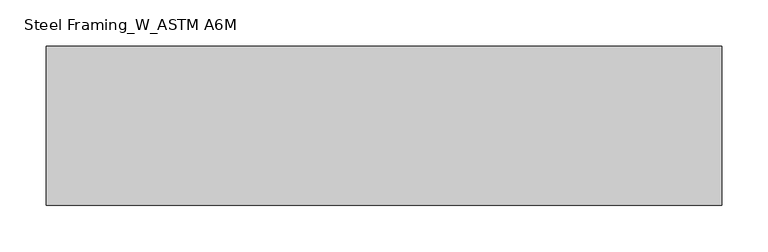
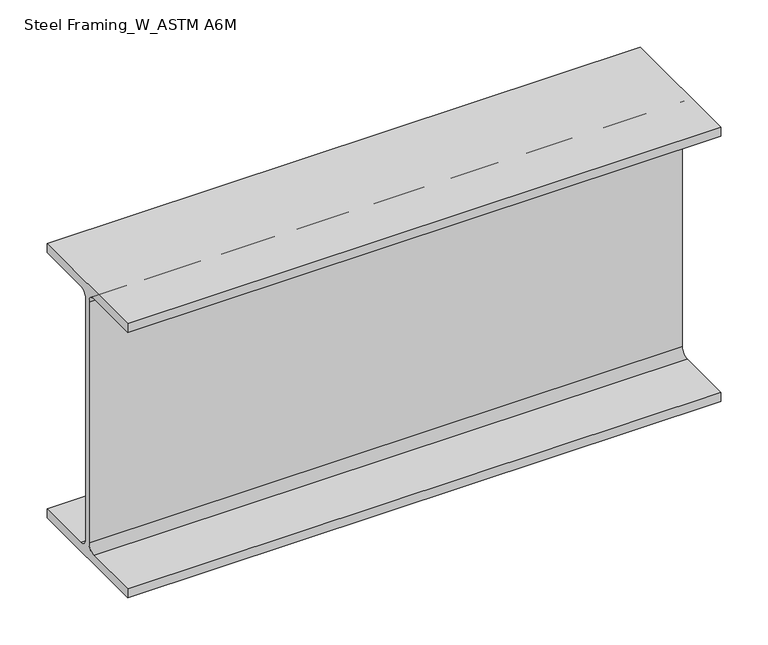
"""IFC4 building model written with IfcOpenShell, lengths in millimetres: beam geometry, Steel Framing_W_ASTM A6M : H_SB_AR_S02_W360x51_RG1."""

import ifcopenshell
import ifcopenshell.guid

model = None  # the IFC model being written
_history = None  # IfcOwnerHistory: only IFC2X3 demands one
_inside = {}  # id of a spatial element -> (the spatial element, [elements in it])
_under = {}  # id of a project, library or spatial element -> (it, [spatial elements below it])
_declared = {}  # id of a project -> (the project, [libraries it declares])
_typed = {}  # id of a type object -> (the type object, [elements of that type])
_made_of = {}  # id of a material, layer set ... -> (it, [elements and type objects made of it])


def new_model(schema):
    """Start an empty IFC model of exactly this schema.

    Asked for "IFC4X3", IfcOpenShell would pick the latest addendum, in which some entities
    have other attributes; the version numbers below select the first issue.
    IFC2X3 requires an IfcOwnerHistory on every rooted entity: one is made here for all.
    """
    global model, _history
    if schema == "IFC4X3":
        model = ifcopenshell.file(schema_version=(4, 3, 0, 0))
    else:
        model = ifcopenshell.file(schema=schema)
    _inside.clear()
    _under.clear()
    _declared.clear()
    _typed.clear()
    _made_of.clear()
    _history = None
    if model.schema == "IFC2X3":
        org = make("IfcOrganization", Name="unknown")
        user = make(
            "IfcPersonAndOrganization",
            ThePerson=make("IfcPerson", FamilyName="unknown"),
            TheOrganization=org,
        )
        app = make(
            "IfcApplication",
            ApplicationDeveloper=org,
            Version="unknown",
            ApplicationFullName="unknown",
            ApplicationIdentifier="unknown",
        )
        _history = make(
            "IfcOwnerHistory",
            OwningUser=user,
            OwningApplication=app,
            ChangeAction="ADDED",
            CreationDate=0,
        )
    return model


def make(cls, **values):
    """One entity of the class cls with the attributes given. An attribute that is None is left unset."""
    return model.create_entity(
        cls, **{name: value for name, value in values.items() if value is not None}
    )


def rooted(cls, **values):
    """An entity with a GlobalId (a new one), such as an element, a storey or a relation."""
    return make(cls, GlobalId=ifcopenshell.guid.new(), OwnerHistory=_history, **values)


def si_unit(unit_type, name, prefix=None):
    """IfcSIUnit, for example si_unit("LENGTHUNIT", "METRE", prefix="MILLI")."""
    return make("IfcSIUnit", UnitType=unit_type, Prefix=prefix, Name=name)


def assignment(units):
    """IfcUnitAssignment: the units of a project."""
    return None if units is None else make("IfcUnitAssignment", Units=units)


def point(xyz):
    """IfcCartesianPoint."""
    return None if xyz is None else make("IfcCartesianPoint", Coordinates=xyz)


def direction(xyz):
    """IfcDirection."""
    return None if xyz is None else make("IfcDirection", DirectionRatios=xyz)


def frame(location, z_axis=None, x_axis=None):
    """IfcAxis2Placement3D, a coordinate frame: its origin and axes. An axis left out is left unset."""
    return make(
        "IfcAxis2Placement3D",
        Location=point(location),
        Axis=direction(z_axis),
        RefDirection=direction(x_axis),
    )


def frame_2d(location, x_axis=None):
    """IfcAxis2Placement2D, a coordinate frame in the plane: its origin and x axis."""
    return make(
        "IfcAxis2Placement2D", Location=point(location), RefDirection=direction(x_axis)
    )


def origin():
    """The frame at (0, 0, 0) with its axes left unset."""
    return frame((0.0, 0.0, 0.0))


def place(relative_to, where):
    """IfcLocalPlacement: puts the frame where relative to a parent placement (None: the world)."""
    return make(
        "IfcLocalPlacement", PlacementRelTo=relative_to, RelativePlacement=where
    )


def context(
    kind, dimensions, precision=None, world=None, true_north=None, identifier=None
):
    """IfcGeometricRepresentationContext, for example the 3D "Model" context."""
    return make(
        "IfcGeometricRepresentationContext",
        ContextIdentifier=identifier,
        ContextType=kind,
        CoordinateSpaceDimension=dimensions,
        Precision=precision,
        WorldCoordinateSystem=world,
        TrueNorth=true_north,
    )


def project(units=None, contexts=None):
    """IfcProject with its units and contexts."""
    return rooted(
        "IfcProject",
        Name="project",
        RepresentationContexts=contexts,
        UnitsInContext=assignment(units),
    )


def spatial(cls, under=None, at=None, **own):
    """A site, building, storey or space (cls), placed at a placement, below another one or the project."""
    s = rooted(cls, ObjectPlacement=at, **own)
    if under is not None:
        _under.setdefault(under.id(), (under, []))[1].append(s)
    return s


def polyline(points):
    """IfcPolyline through the points."""
    return make("IfcPolyline", Points=[point(p) for p in points])


def circle_curve(where, radius):
    """IfcCircle in the frame where."""
    return make("IfcCircle", Position=where, Radius=radius)


def trimmed(basis, trim1, trim2, sense, master):
    """IfcTrimmedCurve: the piece of a basis curve between two trims."""
    return make(
        "IfcTrimmedCurve",
        BasisCurve=basis,
        Trim1=trim1,
        Trim2=trim2,
        SenseAgreement=sense,
        MasterRepresentation=master,
    )


def segment(curve, same_sense, transition):
    """IfcCompositeCurveSegment."""
    return make(
        "IfcCompositeCurveSegment",
        Transition=transition,
        SameSense=same_sense,
        ParentCurve=curve,
    )


def composite_curve(segments, self_intersect=None):
    """IfcCompositeCurve: segments joined end to end."""
    return make("IfcCompositeCurve", Segments=segments, SelfIntersect=self_intersect)


def outline(outer, holes=None, kind="AREA"):
    """IfcArbitraryClosedProfileDef: a profile drawn as a closed curve; with holes, ...WithVoids."""
    if holes is None:
        return make("IfcArbitraryClosedProfileDef", ProfileType=kind, OuterCurve=outer)
    return make(
        "IfcArbitraryProfileDefWithVoids",
        ProfileType=kind,
        OuterCurve=outer,
        InnerCurves=holes,
    )


def extrude(swept, where, along, depth):
    """IfcExtrudedAreaSolid: the profile swept, set in the frame where, extruded along a direction by depth."""
    return make(
        "IfcExtrudedAreaSolid",
        SweptArea=swept,
        Position=where,
        ExtrudedDirection=direction(along),
        Depth=depth,
    )


def shape(context_of_items, identifier, shape_type, items):
    """IfcShapeRepresentation: the items that make up one representation, for example the "Body"."""
    return make(
        "IfcShapeRepresentation",
        ContextOfItems=context_of_items,
        RepresentationIdentifier=identifier,
        RepresentationType=shape_type,
        Items=items,
    )


def source(mapping_origin, context_of_items, identifier, shape_type, items):
    """IfcRepresentationMap: a shape defined once, which mapped items show again and again."""
    return make(
        "IfcRepresentationMap",
        MappingOrigin=mapping_origin,
        MappedRepresentation=shape(context_of_items, identifier, shape_type, items),
    )


def transform(
    local_origin,
    x_axis=None,
    y_axis=None,
    z_axis=None,
    scale=None,
    scale2=None,
    scale3=None,
    uniform=True,
):
    """IfcCartesianTransformationOperator3D, or its non-uniform kind. x_axis, y_axis, z_axis: its Axis1, 2, 3."""
    if uniform:
        return make(
            "IfcCartesianTransformationOperator3D",
            Axis1=direction(x_axis),
            Axis2=direction(y_axis),
            LocalOrigin=point(local_origin),
            Scale=scale,
            Axis3=direction(z_axis),
        )
    return make(
        "IfcCartesianTransformationOperator3DnonUniform",
        Axis1=direction(x_axis),
        Axis2=direction(y_axis),
        LocalOrigin=point(local_origin),
        Scale=scale,
        Axis3=direction(z_axis),
        Scale2=scale2,
        Scale3=scale3,
    )


def mapped(mapping_source, mapping_target):
    """IfcMappedItem: shows the shape of a source again, moved by a transform."""
    return make(
        "IfcMappedItem", MappingSource=mapping_source, MappingTarget=mapping_target
    )


def made_of(thing, what):
    """Note that an element or type object is made of a material, layer set ...; save() writes the relation."""
    if what is not None:
        _made_of.setdefault(what.id(), (what, []))[1].append(thing)
    return thing


def element(
    cls,
    number,
    at=None,
    inside=None,
    cuts=None,
    type_object=None,
    material=None,
    context=None,
    identifier="Body",
    shape_type=None,
    held_by="IfcProductDefinitionShape",
    body=None,
    shapes=None,
    **own,
):
    """One element of the class cls, such as IfcWall. Its Tag is "e" and its number.

    at: its placement. inside: the storey or other place that contains it. cuts: it is an
    opening in that element (IfcRelVoidsElement). A single representation is given by context,
    identifier, shape_type and body (its items); several are given by shapes. held_by: the class
    of the entity that holds the representations. save() writes the other relations.
    """
    e = rooted(cls, Tag="e%d" % number, ObjectPlacement=at, **own)
    if body is not None:
        shapes = [shape(context, identifier, shape_type, body)]
    if shapes is not None:
        e.Representation = make(held_by, Representations=shapes)
    if inside is not None:
        _inside.setdefault(inside.id(), (inside, []))[1].append(e)
    if cuts is not None:
        rooted(
            "IfcRelVoidsElement", RelatingBuildingElement=cuts, RelatedOpeningElement=e
        )
    if type_object is not None:
        _typed.setdefault(type_object.id(), (type_object, []))[1].append(e)
    return made_of(e, material)


def aggregate(whole, parts):
    """IfcRelAggregates: a whole, such as a stair, and the parts it consists of."""
    return rooted("IfcRelAggregates", RelatingObject=whole, RelatedObjects=parts)


def save(model, path):
    """Write the relations noted so far, then the file.

    IfcRelAggregates (storeys below a building ...), IfcRelContainedInSpatialStructure (elements
    in a storey), IfcRelDefinesByType, IfcRelAssociatesMaterial and IfcRelDeclares: one each for
    every whole, place, type object, material and project.
    """
    for whole, parts in _under.values():
        aggregate(whole, parts)
    for where, things in _inside.values():
        rooted(
            "IfcRelContainedInSpatialStructure",
            RelatedElements=things,
            RelatingStructure=where,
        )
    for kind, things in _typed.values():
        rooted("IfcRelDefinesByType", RelatedObjects=things, RelatingType=kind)
    for what, things in _made_of.values():
        rooted("IfcRelAssociatesMaterial", RelatedObjects=things, RelatingMaterial=what)
    for by, libraries in _declared.values():
        rooted("IfcRelDeclares", RelatingContext=by, RelatedDefinitions=libraries)
    model.write(path)


def steel_framing_w_astm_a6m_40fa30bc(model_context):
    return source(origin(), model_context, "Body", "SweptSolid", [
        extrude(outline(composite_curve([segment(polyline([(85.5, -166.4), (85.5, -178.0), (-85.5, -178.0), (-85.5, -166.4), (-13.72, -166.4)]), True, "CONTINUOUS"), segment(trimmed(circle_curve(frame_2d((-13.72, -156.3)), 10.1), [point((-13.72, -166.4))], [point((-3.62, -156.3))], True, "CARTESIAN"), True, "CONTINUOUS"), segment(polyline([(-3.62, -156.3), (-3.62, 156.3)]), True, "CONTINUOUS"), segment(trimmed(circle_curve(frame_2d((-13.72, 156.3)), 10.1), [point((-3.62, 156.3))], [point((-13.72, 166.4))], True, "CARTESIAN"), True, "CONTINUOUS"), segment(polyline([(-13.72, 166.4), (-85.5, 166.4), (-85.5, 178.0), (85.5, 178.0), (85.5, 166.4), (13.72, 166.4)]), True, "CONTINUOUS"), segment(trimmed(circle_curve(frame_2d((13.72, 156.3)), 10.1), [point((13.72, 166.4))], [point((3.62, 156.3))], True, "CARTESIAN"), True, "CONTINUOUS"), segment(polyline([(3.62, 156.3), (3.62, -156.3)]), True, "CONTINUOUS"), segment(trimmed(circle_curve(frame_2d((13.72, -156.3)), 10.1), [point((3.62, -156.3))], [point((13.72, -166.4))], True, "CARTESIAN"), True, "CONTINUOUS"), segment(polyline([(13.72, -166.4), (85.5, -166.4)]), True, "CONTINUOUS")], self_intersect=False)), frame((-228.4, 0.0, 0.0), z_axis=(1.0, 0.0, 0.0), x_axis=(0.0, 1.0, 0.0)), (0.0, 0.0, 1.0), 727.0),
    ])


if __name__ == "__main__":
    model = new_model("IFC4")
    model_context = context("Model", 3, world=origin())
    ifc_project = project(units=[si_unit("LENGTHUNIT", "METRE", prefix="MILLI")], contexts=[model_context])
    site = spatial("IfcSite", under=ifc_project)
    building = spatial("IfcBuilding", under=site)
    placement = place(None, origin())
    steel_framing_w_astm_a6m_shape = steel_framing_w_astm_a6m_40fa30bc(model_context)
    element("IfcBeam", 1, ObjectType="Steel Framing_W_ASTM A6M : H_SB_AR_S02_W360x51_RG1", at=placement, inside=building, context=model_context, shape_type="MappedRepresentation", body=[
        mapped(steel_framing_w_astm_a6m_shape, transform((0.0, 0.0, 0.0), x_axis=(1.0, 0.0, 0.0), y_axis=(0.0, 1.0, 0.0), z_axis=(0.0, 0.0, 1.0))),
    ])
    save(model, "model.ifc")

# Revit data of these elements
# Type "Steel Framing_W_ASTM A6M : H_SB_AR_S02_W360x51_RG1"
#   Type Mark = "RG1"
#   Section Name Key = "W14x34"
#   Width = 17.1 cm
#   Web Thickness = 0.724 cm
#   Web Fillet = 1.01 cm
#   Warping Constant = 287000.0 cm⁶
#   Torsional Moment of Inertia = 23.70 cm⁴
#   Section Area = 64.5 cm²
#   Plastic Modulus weak axis = 174.0 cm³
#   Plastic Modulus strong axis = 895.0 cm³
#   Perimeter = 1.36 m²/m
#   Nominal Weight = 51.00 kgf/m
#   Moment of Inertia weak axis = 970.00 cm⁴
#   Moment of Inertia strong axis = 14200.00 cm⁴
#   Height = 35.6 cm
#   Flange Thickness = 1.16 cm
#   Elastic Modulus weak axis = 113.0 cm³
#   Elastic Modulus strong axis = 796.0 cm³
#   Centroid Vertical = 17.8 cm
#   Centroid Horizontal = 8.55 cm
#   Length [instance default] = 1500 mm
#   Structural Material [instance default] = Steel, 45-345
#   Bolt Spacing = 0
#   Assembly Code = ""
# Element 1 (IfcBeam, "Steel Framing_W_ASTM A6M : H_SB_AR_S02_W360x51_RG1")
#   Materials on its faces: "Steel, 45-345"
# Materials
#   "Steel, 45-345": class "Metal", colour RGB 189 187 185, transparency 0, Description = "Steel 345 MPa", Cost = 0
